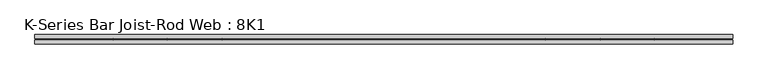
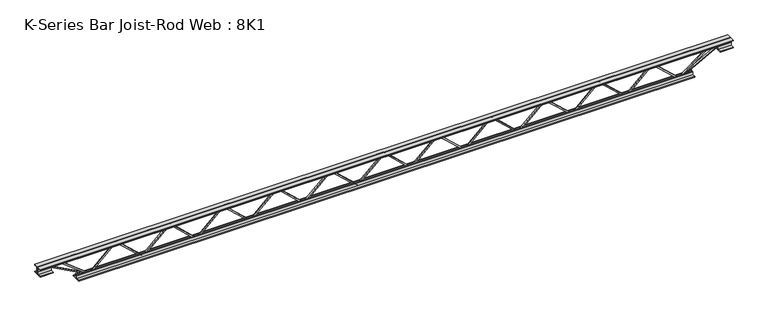
"""IFC4 building model written with IfcOpenShell, lengths in millimetres: beam geometry, K-Series Bar Joist-Rod Web : 8K1."""

from ifc_helpers import new_model, si_unit, frame, origin, place, context, project, spatial, polyline, outline, extrude, source, transform, mapped, element, save


def k_series_bar_joist_rod_web_8k1_7da3c62f(model_context):
    return source(origin(), model_context, "Body", "SweptSolid", [
        extrude(outline(polyline([(-90.4875, 1487.0545455), (-100.0125, 1487.0545455), (-100.0125, 1492.0935213), (90.4875, 1698.1798849), (90.4875, 1700.8019332), (-100.0125, 1906.8882969), (-100.0125, 1911.9272727), (-90.4875, 1911.9272727), (-90.4875, 1910.6162486), (100.0125, 1704.5298849), (100.0125, 1694.4519332), (-90.4875, 1488.3655696), (-90.4875, 1487.0545455)])), frame((0.0, -4.7625, 0.0), z_axis=(0.0, 1.0, 0.0), x_axis=(0.0, 0.0, 1.0)), (0.0, 0.0, 1.0), 9.525),
        extrude(outline(polyline([(-90.4875, 1062.1818182), (-100.0125, 1062.1818182), (-100.0125, 1067.220794), (90.4875, 1273.3071577), (90.4875, 1275.929206), (-100.0125, 1482.0155696), (-100.0125, 1487.0545455), (-90.4875, 1487.0545455), (-90.4875, 1485.7435213), (100.0125, 1279.6571577), (100.0125, 1269.579206), (-90.4875, 1063.4928423), (-90.4875, 1062.1818182)])), frame((0.0, -4.7625, 0.0), z_axis=(0.0, 1.0, 0.0), x_axis=(0.0, 0.0, 1.0)), (0.0, 0.0, 1.0), 9.525),
        extrude(outline(polyline([(-90.4875, 637.3090909), (-100.0125, 637.3090909), (-100.0125, 642.3480668), (90.4875, 848.4344304), (90.4875, 851.0564787), (-100.0125, 1057.1428423), (-100.0125, 1062.1818182), (-90.4875, 1062.1818182), (-90.4875, 1060.870794), (100.0125, 854.7844304), (100.0125, 844.7064787), (-90.4875, 638.6201151), (-90.4875, 637.3090909)])), frame((0.0, -4.7625, 0.0), z_axis=(0.0, 1.0, 0.0), x_axis=(0.0, 0.0, 1.0)), (0.0, 0.0, 1.0), 9.525),
        extrude(outline(polyline([(-90.4875, 212.4363636), (-100.0125, 212.4363636), (-100.0125, 217.4753395), (90.4875, 423.5617031), (90.4875, 426.1837514), (-100.0125, 632.2701151), (-100.0125, 637.3090909), (-90.4875, 637.3090909), (-90.4875, 635.9980668), (100.0125, 429.9117031), (100.0125, 419.8337514), (-90.4875, 213.7473878), (-90.4875, 212.4363636)])), frame((0.0, -4.7625, 0.0), z_axis=(0.0, 1.0, 0.0), x_axis=(0.0, 0.0, 1.0)), (0.0, 0.0, 1.0), 9.525),
        extrude(outline(polyline([(-90.4875, -212.4363636), (-100.0125, -212.4363636), (-100.0125, -207.3973878), (90.4875, -1.3110241), (90.4875, 1.3110241), (-100.0125, 207.3973878), (-100.0125, 212.4363636), (-90.4875, 212.4363636), (-90.4875, 211.1253395), (100.0125, 5.0389759), (100.0125, -5.0389759), (-90.4875, -211.1253395), (-90.4875, -212.4363636)])), frame((0.0, -4.7625, 0.0), z_axis=(0.0, 1.0, 0.0), x_axis=(0.0, 0.0, 1.0)), (0.0, 0.0, 1.0), 9.525),
        extrude(outline(polyline([(-90.4875, -637.3090909), (-100.0125, -637.3090909), (-100.0125, -632.2701151), (90.4875, -426.1837514), (90.4875, -423.5617031), (-100.0125, -217.4753395), (-100.0125, -212.4363636), (-90.4875, -212.4363636), (-90.4875, -213.7473878), (100.0125, -419.8337514), (100.0125, -429.9117031), (-90.4875, -635.9980668), (-90.4875, -637.3090909)])), frame((0.0, -4.7625, 0.0), z_axis=(0.0, 1.0, 0.0), x_axis=(0.0, 0.0, 1.0)), (0.0, 0.0, 1.0), 9.525),
        extrude(outline(polyline([(-90.4875, -1062.1818182), (-100.0125, -1062.1818182), (-100.0125, -1057.1428423), (90.4875, -851.0564787), (90.4875, -848.4344304), (-100.0125, -642.3480668), (-100.0125, -637.3090909), (-90.4875, -637.3090909), (-90.4875, -638.6201151), (100.0125, -844.7064787), (100.0125, -854.7844304), (-90.4875, -1060.870794), (-90.4875, -1062.1818182)])), frame((0.0, -4.7625, 0.0), z_axis=(0.0, 1.0, 0.0), x_axis=(0.0, 0.0, 1.0)), (0.0, 0.0, 1.0), 9.525),
        extrude(outline(polyline([(-90.4875, -1487.0545455), (-100.0125, -1487.0545455), (-100.0125, -1482.0155696), (90.4875, -1275.929206), (90.4875, -1273.3071577), (-100.0125, -1067.220794), (-100.0125, -1062.1818182), (-90.4875, -1062.1818182), (-90.4875, -1063.4928423), (100.0125, -1269.579206), (100.0125, -1279.6571577), (-90.4875, -1485.7435213), (-90.4875, -1487.0545455)])), frame((0.0, -4.7625, 0.0), z_axis=(0.0, 1.0, 0.0), x_axis=(0.0, 0.0, 1.0)), (0.0, 0.0, 1.0), 9.525),
        extrude(outline(polyline([(-90.4875, -1911.9272727), (-100.0125, -1911.9272727), (-100.0125, -1906.8882969), (90.4875, -1700.8019332), (90.4875, -1698.1798849), (-100.0125, -1492.0935213), (-100.0125, -1487.0545455), (-90.4875, -1487.0545455), (-90.4875, -1488.3655696), (100.0125, -1694.4519332), (100.0125, -1704.5298849), (-90.4875, -1910.6162486), (-90.4875, -1911.9272727)])), frame((0.0, -4.7625, 0.0), z_axis=(0.0, 1.0, 0.0), x_axis=(0.0, 0.0, 1.0)), (0.0, 0.0, 1.0), 9.525),
        extrude(outline(polyline([(-90.4875, 1911.9272727), (-100.0125, 1911.9272727), (-100.0125, 1916.9662486), (90.4875, 2123.0526122), (90.4875, 2125.6746605), (-100.0125, 2331.7610241), (-100.0125, 2336.8), (-90.4875, 2336.8), (-90.4875, 2335.4889759), (100.0125, 2129.4026122), (100.0125, 2119.3246605), (-90.4875, 1913.2382969), (-90.4875, 1911.9272727)])), frame((0.0, -4.7625, 0.0), z_axis=(0.0, 1.0, 0.0), x_axis=(0.0, 0.0, 1.0)), (0.0, 0.0, 1.0), 9.525),
        extrude(outline(polyline([(-90.4875, -2336.8), (-100.0125, -2336.8), (-100.0125, -2331.7610241), (90.4875, -2125.6746605), (90.4875, -2123.0526122), (-100.0125, -1916.9662486), (-100.0125, -1911.9272727), (-90.4875, -1911.9272727), (-90.4875, -1913.2382969), (100.0125, -2119.3246605), (100.0125, -2129.4026122), (-90.4875, -2335.4889759), (-90.4875, -2336.8)])), frame((0.0, -4.7625, 0.0), z_axis=(0.0, 1.0, 0.0), x_axis=(0.0, 0.0, 1.0)), (0.0, 0.0, 1.0), 9.525),
        extrude(outline(polyline([(4.7625, 101.6), (36.5125, 101.6), (36.5125, 95.25), (11.1125, 95.25), (11.1125, 69.85), (4.7625, 69.85), (4.7625, 101.6)])), frame((-2743.2, 0.0, 0.0), z_axis=(1.0, 0.0, 0.0), x_axis=(0.0, 1.0, 0.0)), (0.0, 0.0, 1.0), 5486.4),
        extrude(outline(polyline([(-4.7625, 101.6), (-4.7625, 69.85), (-11.1125, 69.85), (-11.1125, 95.25), (-36.5125, 95.25), (-36.5125, 101.6), (-4.7625, 101.6)])), frame((-2743.2, 0.0, 0.0), z_axis=(1.0, 0.0, 0.0), x_axis=(0.0, 1.0, 0.0)), (0.0, 0.0, 1.0), 5486.4),
        extrude(outline(polyline([(-4.7625, 38.1), (-36.5125, 38.1), (-36.5125, 44.45), (-11.1125, 44.45), (-11.1125, 69.85), (-4.7625, 69.85), (-4.7625, 38.1)])), frame((-2743.2, 0.0, 0.0), z_axis=(1.0, 0.0, 0.0), x_axis=(0.0, 1.0, 0.0)), (0.0, 0.0, 1.0), 101.6),
        extrude(outline(polyline([(36.5125, 38.1), (4.7625, 38.1), (4.7625, 69.85), (11.1125, 69.85), (11.1125, 44.45), (36.5125, 44.45), (36.5125, 38.1)])), frame((-2743.2, 0.0, 0.0), z_axis=(1.0, 0.0, 0.0), x_axis=(0.0, 1.0, 0.0)), (0.0, 0.0, 1.0), 101.6),
        extrude(outline(polyline([(4.7625, 38.1), (4.7625, 69.85), (11.1125, 69.85), (11.1125, 44.45), (36.5125, 44.45), (36.5125, 38.1), (4.7625, 38.1)])), frame((2641.6, 0.0, 0.0), z_axis=(1.0, 0.0, 0.0), x_axis=(0.0, 1.0, 0.0)), (0.0, 0.0, 1.0), 101.6),
        extrude(outline(polyline([(-4.7625, 38.1), (-36.5125, 38.1), (-36.5125, 44.45), (-11.1125, 44.45), (-11.1125, 69.85), (-4.7625, 69.85), (-4.7625, 38.1)])), frame((2641.6, 0.0, 0.0), z_axis=(1.0, 0.0, 0.0), x_axis=(0.0, 1.0, 0.0)), (0.0, 0.0, 1.0), 101.6),
        extrude(outline(polyline([(4.7625, -101.6), (4.7625, -69.85), (11.1125, -69.85), (11.1125, -95.25), (36.5125, -95.25), (36.5125, -101.6), (4.7625, -101.6)])), frame((-2438.4, 0.0, 0.0), z_axis=(1.0, 0.0, 0.0), x_axis=(0.0, 1.0, 0.0)), (0.0, 0.0, 1.0), 4876.8),
        extrude(outline(polyline([(-4.7625, -101.6), (-36.5125, -101.6), (-36.5125, -95.25), (-11.1125, -95.25), (-11.1125, -69.85), (-4.7625, -69.85), (-4.7625, -101.6)])), frame((-2438.4, 0.0, 0.0), z_axis=(1.0, 0.0, 0.0), x_axis=(0.0, 1.0, 0.0)), (0.0, 0.0, 1.0), 4876.8),
        extrude(outline(polyline([(0.0, -9.525), (0.0, 0.0), (346.6425392, 0.0), (346.6425392, -9.525), (0.0, -9.525)])), frame((-2643.8682985, 4.7625, 65.662372), z_axis=(0.4762831485400797, 0.0, 0.8792919665371386), x_axis=(0.8792919665371386, 0.0, -0.4762831485400797)), (0.0, 0.0, 1.0), 9.525),
        extrude(outline(polyline([(0.0, -9.525), (0.0, 0.0), (269.048729, 0.0), (269.048729, -9.525), (0.0, -9.525)])), frame((-2552.1588407, 4.7625, 66.0896099), z_axis=(0.6136434860418419, 0.0, 0.7895832267965269), x_axis=(0.7895832267965269, 0.0, -0.6136434860418419)), (0.0, 0.0, 1.0), 9.525),
        extrude(outline(polyline([(0.0, -9.525), (0.0, 0.0), (346.6425392, 0.0), (346.6425392, -9.525), (0.0, -9.525)])), frame((2643.8682985, -4.7625, 65.662372), z_axis=(-0.4762831485400416, 0.0, 0.8792919665371592), x_axis=(-0.8792919665371592, 0.0, -0.4762831485400416)), (0.0, 0.0, 1.0), 9.525),
        extrude(outline(polyline([(0.0, -9.525), (0.0, 0.0), (269.048729, 0.0), (269.048729, -9.525), (0.0, -9.525)])), frame((2552.1588407, -4.7625, 66.0896099), z_axis=(-0.6136434860418192, 0.0, 0.7895832267965447), x_axis=(-0.7895832267965447, 0.0, -0.6136434860418192)), (0.0, 0.0, 1.0), 9.525),
    ])


if __name__ == "__main__":
    model = new_model("IFC4")
    model_context = context("Model", 3, world=origin())
    ifc_project = project(units=[si_unit("LENGTHUNIT", "METRE", prefix="MILLI")], contexts=[model_context])
    site = spatial("IfcSite", under=ifc_project)
    building = spatial("IfcBuilding", under=site)
    placement = place(None, origin())
    k_series_bar_joist_rod_web_8k1_shape = k_series_bar_joist_rod_web_8k1_7da3c62f(model_context)
    element("IfcBeam", 1, ObjectType="K-Series Bar Joist-Rod Web : 8K1", at=placement, inside=building, context=model_context, shape_type="MappedRepresentation", body=[
        mapped(k_series_bar_joist_rod_web_8k1_shape, transform((0.0, 0.0, 0.0), x_axis=(1.0, 0.0, 0.0), y_axis=(0.0, 1.0, 0.0), z_axis=(0.0, 0.0, 1.0))),
    ])
    save(model, "model.ifc")

# Revit data of these elements
# Type "K-Series Bar Joist-Rod Web : 8K1"
#   Assembly Code = "B1010350"
#   Wt = 5.1
#   Web Thickness = 0' - 0 3/8"
#   Start Offset [instance default] = 0' - 0"
#   Start Extension [instance default] = 0' - 0"
#   Seat Length = 0' - 4"
#   Seat Depth = 0' - 2 1/2"
#   PanelArrayLength [instance default] = 21' - 4"
#   Panel [instance default] = 1' - 4"
#   End Offset [instance default] = 0' - 0"
#   End Extension [instance default] = 0' - 0"
#   End Panel = 1' - 4"
#   Cord Leg = 0' - 1 1/4"
#   Chord Thickness = 0' - 0 1/4"
#   Length [instance default] = 24' - 0"
#   Depth = 0' - 8"
#   PanelArrayNum [instance default] = 16
#   Rendering Material = none
# Element 1 (IfcBeam, "K-Series Bar Joist-Rod Web : 8K1")
#   PanelArrayLength = 15' - 4"
#   Panel = 1' - 4.72727"
#   PanelArrayNum = 11
